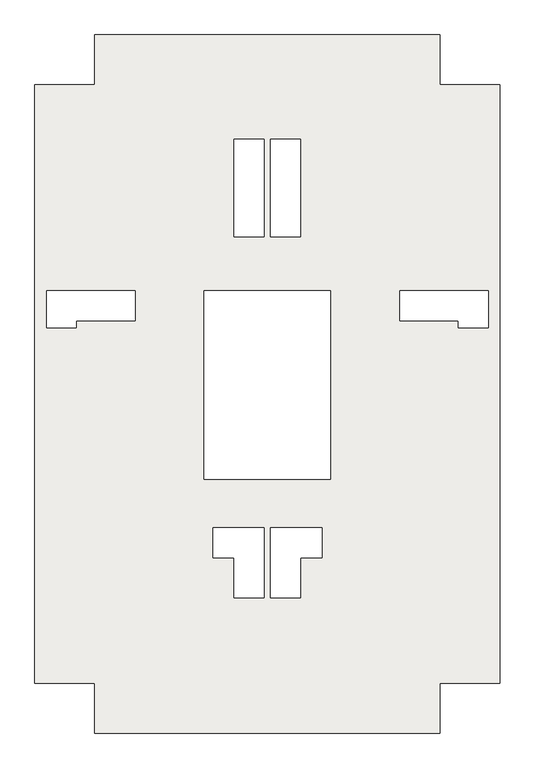
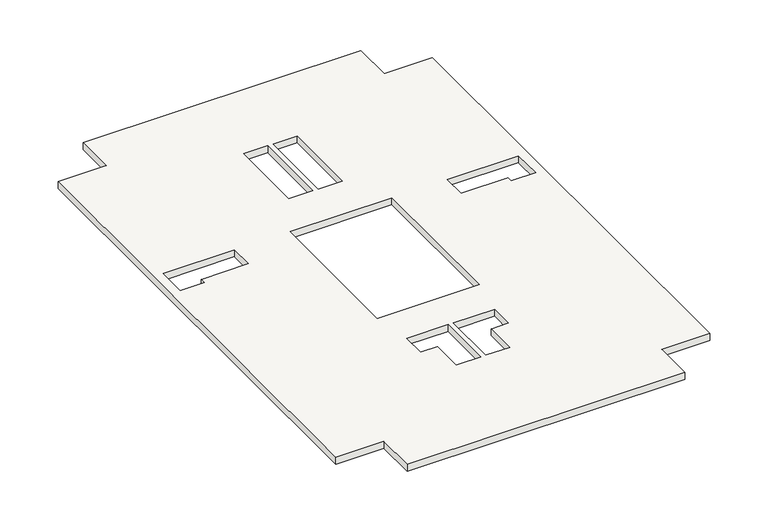
"""IFC4 building model written with IfcOpenShell, lengths in millimetres: slab geometry, Holzdecke."""

from ifc_helpers import new_model, si_unit, origin, origin_with_axes, place, context, project, spatial, polyline, outline, extrude, source, transform, mapped, element, save


def slab_a8e48092(model_context):
    return source(origin(), model_context, "Body", "SweptSolid", [
        extrude(outline(polyline([(1800.0, 1500.0), (0.0, 1500.0), (0.0, 19502.8619019), (1800.0, 19502.8619019), (1800.0, 21002.8619019), (12200.0, 21002.8619019), (12200.0, 19502.8619019), (14000.0, 19502.8619019), (14000.0, 1500.0), (12200.0, 1500.0), (12200.0, 0.0), (1800.0, 0.0), (1800.0, 1500.0)]), holes=[polyline([(3014.6018366, 12402.8619019), (3014.6018366, 13302.8619019), (350.0, 13302.8619019), (350.0, 12198.126196), (1250.0, 12198.126196), (1250.0, 12402.8619019), (3014.6018366, 12402.8619019)]), polyline([(7100.0, 6177.8619019), (7100.0, 4073.2600653), (8000.0, 4073.2600653), (8000.0, 5277.8619019), (8640.0, 5277.8619019), (8640.0, 6177.8619019), (7100.0, 6177.8619019)]), polyline([(5360.0, 5277.8619019), (6000.0, 5277.8619019), (6000.0, 4073.2600653), (6900.0, 4073.2600653), (6900.0, 6177.8619019), (5360.0, 6177.8619019), (5360.0, 5277.8619019)]), polyline([(12750.0, 12402.8619019), (12750.0, 12198.126196), (13650.0, 12198.126196), (13650.0, 13302.8619019), (10985.3981634, 13302.8619019), (10985.3981634, 12402.8619019), (12750.0, 12402.8619019)]), polyline([(8000.0, 17860.6619019), (7100.0, 17860.6619019), (7100.0, 14932.8619019), (8000.0, 14932.8619019), (8000.0, 17860.6619019)]), polyline([(6000.0, 14932.8619019), (6900.0, 14932.8619019), (6900.0, 17860.6619019), (6000.0, 17860.6619019), (6000.0, 14932.8619019)]), polyline([(5100.0, 13302.8619019), (5100.0, 7632.8619019), (8900.0, 7632.8619019), (8900.0, 13302.8619019), (5100.0, 13302.8619019)])]), origin_with_axes(), (0.0, 0.0, 1.0), 270.0),
    ])


if __name__ == "__main__":
    model = new_model("IFC4")
    model_context = context("Model", 3, world=origin())
    ifc_project = project(units=[si_unit("LENGTHUNIT", "METRE", prefix="MILLI")], contexts=[model_context])
    site = spatial("IfcSite", under=ifc_project)
    building = spatial("IfcBuilding", under=site)
    placement = place(None, origin())
    slab_shape = slab_a8e48092(model_context)
    element("IfcSlab", 1, ObjectType="Holzdecke", at=placement, inside=building, context=model_context, shape_type="MappedRepresentation", body=[
        mapped(slab_shape, transform((0.0, 0.0, 0.0), x_axis=(1.0, 0.0, 0.0), y_axis=(0.0, 1.0, 0.0), z_axis=(0.0, 0.0, 1.0))),
    ])
    save(model, "model.ifc")

# Revit data of these elements
# Element 1 (IfcSlab, "Holzdecke")
#   Materials on its faces: "holzschalung"
# Materials
#   "holzschalung": class "Unassigned", colour RGB 128 128 128, transparency 0
